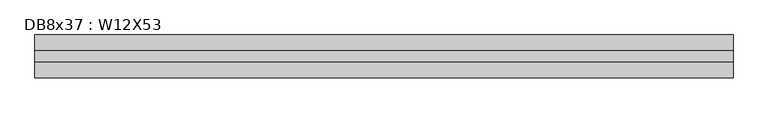
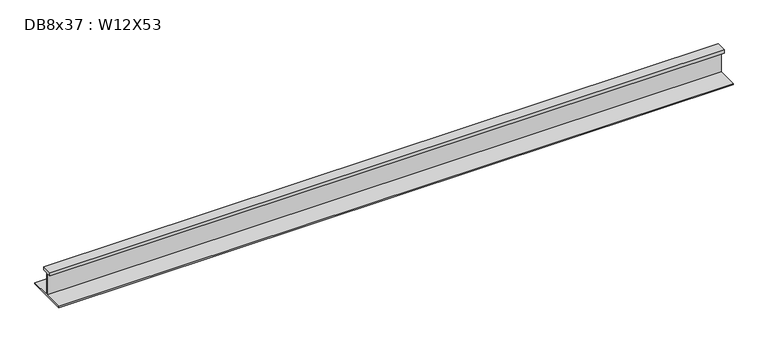
"""IFC4 building model written with IfcOpenShell, lengths in millimetres: beam geometry, DB8x37 : W12X53."""

from ifc_helpers import new_model, si_unit, frame, origin, place, context, project, spatial, polyline, outline, extrude, source, transform, mapped, element, save


def db8x37_w12x53_0a7cf7c0(model_context):
    return source(origin(), model_context, "Body", "SweptSolid", [
        extrude(outline(polyline([(38.1, 145.415), (38.1, 120.015), (2.921, 120.015), (2.921, -48.4505), (152.4, -48.4505), (152.4, -58.1025), (-152.4, -58.1025), (-152.4, -48.4505), (-2.921, -48.4505), (-2.921, 120.015), (-38.1, 120.015), (-38.1, 145.415), (38.1, 145.415)])), frame((-2479.929, 0.0, 0.0), z_axis=(1.0, 0.0, 0.0), x_axis=(0.0, 1.0, 0.0)), (0.0, 0.0, 1.0), 4959.858),
    ])


if __name__ == "__main__":
    model = new_model("IFC4")
    model_context = context("Model", 3, world=origin())
    ifc_project = project(units=[si_unit("LENGTHUNIT", "METRE", prefix="MILLI")], contexts=[model_context])
    site = spatial("IfcSite", under=ifc_project)
    building = spatial("IfcBuilding", under=site)
    placement = place(None, origin())
    db8x37_w12x53_shape = db8x37_w12x53_0a7cf7c0(model_context)
    element("IfcBeam", 1, ObjectType="DB8x37 : W12X53", at=placement, inside=building, context=model_context, shape_type="MappedRepresentation", body=[
        mapped(db8x37_w12x53_shape, transform((0.0, 0.0, 0.0), x_axis=(1.0, 0.0, 0.0), y_axis=(0.0, 1.0, 0.0), z_axis=(0.0, 0.0, 1.0))),
    ])
    save(model, "model.ifc")

# Revit data of these elements
# Type "DB8x37 : W12X53"
#   Assembly Code = "B10"
#   W = 53
#   Length [instance default] = 5' - 0"
#   bf = 0' - 10"
#   d = 1' - 0.1"
#   k = 0' - 1 3/8"
#   k2 = 0' - 0.8"
#   tf = 0' - 0.575"
#   tw = 0' - 0.345"
#   A = 0.108333 SF
#   Structural Material [instance default] = Steel ASTM A992
# Element 1 (IfcBeam, "DB8x37 : W12X53")
#   Materials on its faces: "Steel ASTM A992"
# Materials
#   "Steel ASTM A992": class "Metal", colour RGB 199 199 199, transparency 0, Description = "Structural steel 50ksi", Cost = 0
